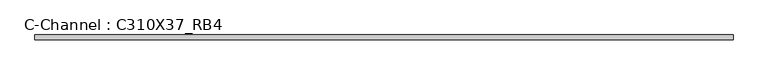
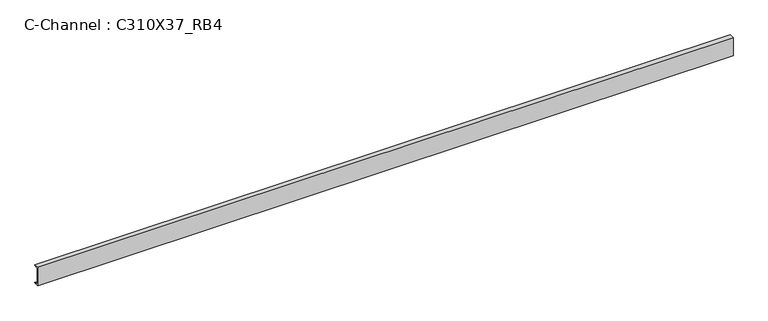
"""IFC4 building model written with IfcOpenShell, lengths in millimetres: beam geometry, C-Channel : C310X37_RB4."""

from ifc_helpers import new_model, si_unit, point, frame, frame_2d, origin, place, context, project, spatial, polyline, circle_curve, trimmed, segment, composite_curve, outline, extrude, source, transform, mapped, element, save


def c_channel_c310x37_rb4_366fd90e(model_context):
    return source(origin(), model_context, "Body", "SweptSolid", [
        extrude(outline(composite_curve([segment(polyline([(-17.1196, 152.4), (60.3504, 152.4)]), True, "CONTINUOUS"), segment(trimmed(circle_curve(frame_2d((47.625, 152.4)), 12.7254), [point((60.3504, 152.4))], [point((47.625, 139.6746))], False, "CARTESIAN"), True, "CONTINUOUS"), segment(polyline([(47.625, 139.6746), (-7.2898, 130.9769501), (-7.2898, -130.9769501), (47.625, -139.6746)]), True, "CONTINUOUS"), segment(trimmed(circle_curve(frame_2d((47.625, -152.4)), 12.7254), [point((47.625, -139.6746))], [point((60.3504, -152.4))], False, "CARTESIAN"), True, "CONTINUOUS"), segment(polyline([(60.3504, -152.4), (-17.1196, -152.4), (-17.1196, 152.4)]), True, "CONTINUOUS")], self_intersect=False)), frame((-5534.2426351, 0.0, 0.0), z_axis=(1.0, 0.0, 0.0), x_axis=(0.0, 1.0, 0.0)), (0.0, 0.0, 1.0), 11047.2668415),
    ])


if __name__ == "__main__":
    model = new_model("IFC4")
    model_context = context("Model", 3, world=origin())
    ifc_project = project(units=[si_unit("LENGTHUNIT", "METRE", prefix="MILLI")], contexts=[model_context])
    site = spatial("IfcSite", under=ifc_project)
    building = spatial("IfcBuilding", under=site)
    placement = place(None, origin())
    c_channel_c310x37_rb4_shape = c_channel_c310x37_rb4_366fd90e(model_context)
    element("IfcBeam", 1, ObjectType="C-Channel : C310X37_RB4", at=placement, inside=building, context=model_context, shape_type="MappedRepresentation", body=[
        mapped(c_channel_c310x37_rb4_shape, transform((0.0, 0.0, 0.0), x_axis=(1.0, 0.0, 0.0), y_axis=(0.0, 1.0, 0.0), z_axis=(0.0, 0.0, 1.0))),
    ])
    save(model, "model.ifc")

# Revit data of these elements
# Type "C-Channel : C310X37_RB4"
#   Assembly Code = "B10"
#   W = 25
#   Length [instance default] = 1524 mm
#   bf = 77.47 mm
#   d = 304.8 mm
#   tf = 12.725 mm
#   tw = 9.83 mm
#   x = 17.12 mm
#   A = 0.00473547 m²
#   Structural Material [instance default] = Steel ASTM A36
# Element 1 (IfcBeam, "C-Channel : C310X37_RB4")
#   Structural Material = Steel ASTM A992
#   Materials on its faces: "Steel ASTM A992"
# Materials
#   "Steel ASTM A36": class "Metal", colour RGB 199 199 199, transparency 0, Description = "Structural steel, ASTM A36 Grade B, mill finish", Cost = 0
#   "Steel ASTM A992": class "Metal", colour RGB 199 199 199, transparency 0, Description = "Structural steel 50ksi", Cost = 0
